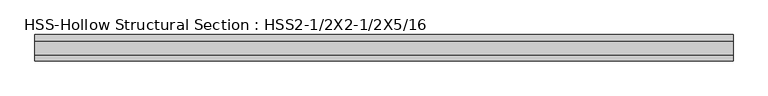
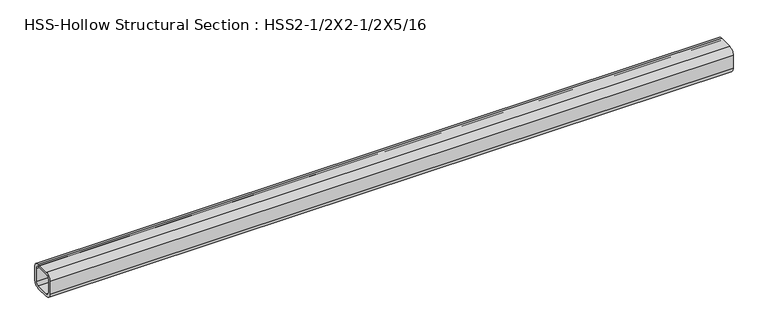
"""IFC4 building model written with IfcOpenShell, lengths in millimetres: beam geometry, HSS-Hollow Structural Section : HSS2-1/2X2-1/2X5/16."""

from ifc_helpers import new_model, si_unit, point, frame, frame_2d, origin, place, context, project, spatial, polyline, circle_curve, trimmed, segment, composite_curve, outline, extrude, source, transform, mapped, element, save


def hss_hollow_structural_section_hss2_1_2x2_1_2x5_16_05f66c46(model_context):
    return source(origin(), model_context, "Body", "SweptSolid", [
        extrude(outline(composite_curve([segment(polyline([(31.75, 16.9672), (31.75, -16.9672)]), True, "CONTINUOUS"), segment(trimmed(circle_curve(frame_2d((16.9672, -16.9672)), 14.7828), [point((31.75, -16.9672))], [point((16.9672, -31.75))], False, "CARTESIAN"), True, "CONTINUOUS"), segment(polyline([(16.9672, -31.75), (-16.9672, -31.75)]), True, "CONTINUOUS"), segment(trimmed(circle_curve(frame_2d((-16.9672, -16.9672)), 14.7828), [point((-16.9672, -31.75))], [point((-31.75, -16.9672))], False, "CARTESIAN"), True, "CONTINUOUS"), segment(polyline([(-31.75, -16.9672), (-31.75, 16.9672)]), True, "CONTINUOUS"), segment(trimmed(circle_curve(frame_2d((-16.9672, 16.9672)), 14.7828), [point((-31.75, 16.9672))], [point((-16.9672, 31.75))], False, "CARTESIAN"), True, "CONTINUOUS"), segment(polyline([(-16.9672, 31.75), (16.9672, 31.75)]), True, "CONTINUOUS"), segment(trimmed(circle_curve(frame_2d((16.9672, 16.9672)), 14.7828), [point((16.9672, 31.75))], [point((31.75, 16.9672))], False, "CARTESIAN"), True, "CONTINUOUS")], self_intersect=False), holes=[composite_curve([segment(trimmed(circle_curve(frame_2d((-16.9672, 16.9672)), 7.3914), [point((-16.9672, 24.3586))], [point((-24.3586, 16.9672))], True, "CARTESIAN"), True, "CONTINUOUS"), segment(polyline([(-24.3586, 16.9672), (-24.3586, -16.9672)]), True, "CONTINUOUS"), segment(trimmed(circle_curve(frame_2d((-16.9672, -16.9672)), 7.3914), [point((-24.3586, -16.9672))], [point((-16.9672, -24.3586))], True, "CARTESIAN"), True, "CONTINUOUS"), segment(polyline([(-16.9672, -24.3586), (16.9672, -24.3586)]), True, "CONTINUOUS"), segment(trimmed(circle_curve(frame_2d((16.9672, -16.9672)), 7.3914), [point((16.9672, -24.3586))], [point((24.3586, -16.9672))], True, "CARTESIAN"), True, "CONTINUOUS"), segment(polyline([(24.3586, -16.9672), (24.3586, 16.9672)]), True, "CONTINUOUS"), segment(trimmed(circle_curve(frame_2d((16.9672, 16.9672)), 7.3914), [point((24.3586, 16.9672))], [point((16.9672, 24.3586))], True, "CARTESIAN"), True, "CONTINUOUS"), segment(polyline([(16.9672, 24.3586), (-16.9672, 24.3586)]), True, "CONTINUOUS")], self_intersect=False)]), frame((-831.85, 0.0, 0.0), z_axis=(1.0, 0.0, 0.0), x_axis=(0.0, 1.0, 0.0)), (0.0, 0.0, 1.0), 1682.623),
    ])


if __name__ == "__main__":
    model = new_model("IFC4")
    model_context = context("Model", 3, world=origin())
    ifc_project = project(units=[si_unit("LENGTHUNIT", "METRE", prefix="MILLI")], contexts=[model_context])
    site = spatial("IfcSite", under=ifc_project)
    building = spatial("IfcBuilding", under=site)
    placement = place(None, origin())
    hss_hollow_structural_section_hss2_1_2x2_1_2x5_16_shape = hss_hollow_structural_section_hss2_1_2x2_1_2x5_16_05f66c46(model_context)
    element("IfcBeam", 1, ObjectType="HSS-Hollow Structural Section : HSS2-1/2X2-1/2X5/16", at=placement, inside=building, context=model_context, shape_type="MappedRepresentation", body=[
        mapped(hss_hollow_structural_section_hss2_1_2x2_1_2x5_16_shape, transform((0.0, 0.0, 0.0), x_axis=(1.0, 0.0, 0.0), y_axis=(0.0, 1.0, 0.0), z_axis=(0.0, 0.0, 1.0))),
    ])
    save(model, "model.ifc")

# Revit data of these elements
# Type "HSS-Hollow Structural Section : HSS2-1/2X2-1/2X5/16"
#   Assembly Code = "B10"
#   Shape = "Square"
#   W = 8.4
#   Ht = 0' - 2 1/2"
#   Length [instance default] = 5' - 0"
#   b = 0' - 2 1/2"
#   kr = 0' - 0.582"
#   t = 0' - 0.291"
#   A = 0.0163194 SF
#   Structural Material [instance default] = Steel ASTM A500, Grade B, Rectangular and Square
# Element 1 (IfcBeam, "HSS-Hollow Structural Section : HSS2-1/2X2-1/2X5/16")
#   Materials on its faces: "Steel ASTM A500, Grade B, Rectangular and Square"
# Materials
#   "Steel ASTM A500, Grade B, Rectangular and Square": class "Metal", colour RGB 199 199 199, transparency 0, Description = "Carbon steel", Cost = 0
